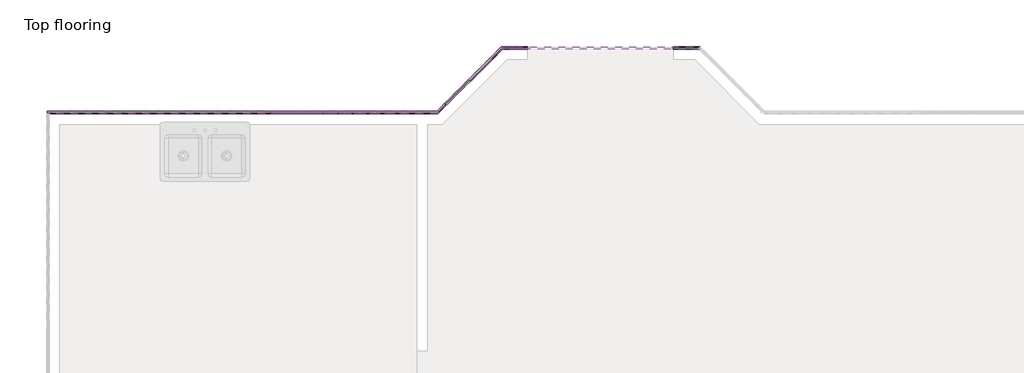
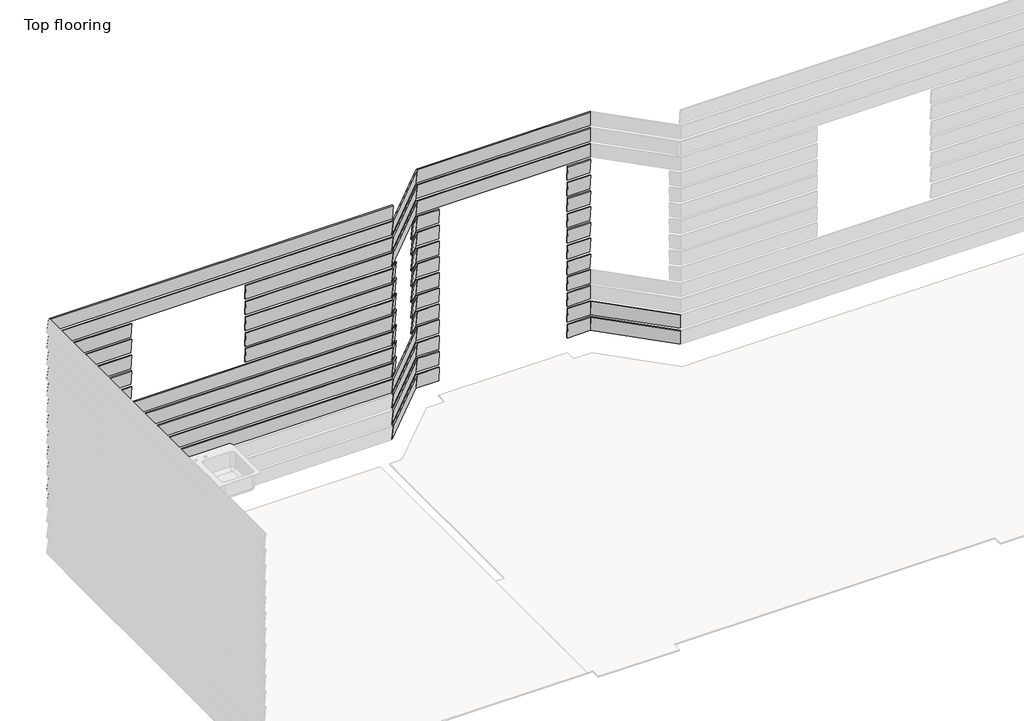
# One storey, part 4 of 5: 42 proxies.
"""IFC4 building model written with IfcOpenShell, lengths in millimetres."""

from ifc_helpers import new_model, si_unit, origin, place, context, project, spatial, faceted_brep, element, save

model = new_model("IFC4")

# Units and contexts
model_context = context("Model", 3, world=origin())
ifc_project = project(units=[si_unit("LENGTHUNIT", "METRE", prefix="MILLI")], contexts=[model_context])

# Site, building, storey
site = spatial("IfcSite", under=ifc_project)
building = spatial("IfcBuilding", under=site)
storey = spatial("IfcBuildingStorey", under=building, Name="Top flooring", Elevation=12.7)

# Proxies
placement = place(None, origin())
element("IfcBuildingElementProxy", 1, Name="Wall Sweeps", at=placement, inside=storey, context=model_context, shape_type="Brep", body=[
    faceted_brep([(-14153.612325, 5231.8645018, 179.3151454), (-14149.4864779, 5221.9038257, 178.429182), (-14143.614829, 5207.7284114, 337.8), (-14147.7406762, 5217.6890875, 338.6859634), (-13544.012325, 5841.4645018, 179.3151454), (-13538.1406762, 5827.2890875, 338.6859634), (-13534.014829, 5817.3284114, 337.8), (-13539.8864779, 5831.5038257, 178.429182)], [[[0, 1, 2, 3]], [[4, 5, 6, 7]], [[1, 0, 4, 7]], [[2, 1, 7, 6]], [[3, 2, 6, 5]], [[0, 3, 5, 4]]]),
])
element("IfcBuildingElementProxy", 2, Name="Wall Sweeps", at=placement, inside=storey, context=model_context, shape_type="Brep", body=[
    faceted_brep([(-14153.612325, 5231.8645018, 357.1151454), (-14149.4864779, 5221.9038257, 356.229182), (-14143.614829, 5207.7284114, 515.6), (-14147.7406762, 5217.6890875, 516.4859634), (-13544.012325, 5841.4645018, 357.1151454), (-13538.1406762, 5827.2890875, 516.4859634), (-13534.014829, 5817.3284114, 515.6), (-13539.8864779, 5831.5038257, 356.229182)], [[[0, 1, 2, 3]], [[4, 5, 6, 7]], [[1, 0, 4, 7]], [[2, 1, 7, 6]], [[3, 2, 6, 5]], [[0, 3, 5, 4]]]),
])
element("IfcBuildingElementProxy", 3, Name="Wall Sweeps", at=placement, inside=storey, context=model_context, shape_type="Brep", body=[
    faceted_brep([(-14153.612325, 5231.8645018, 534.9151454), (-14149.4864779, 5221.9038257, 534.029182), (-14143.614829, 5207.7284114, 693.4), (-14147.7406762, 5217.6890875, 694.2859634), (-13544.012325, 5841.4645018, 534.9151454), (-13538.1406762, 5827.2890875, 694.2859634), (-13534.014829, 5817.3284114, 693.4), (-13539.8864779, 5831.5038257, 534.029182)], [[[0, 1, 2, 3]], [[4, 5, 6, 7]], [[1, 0, 4, 7]], [[2, 1, 7, 6]], [[3, 2, 6, 5]], [[0, 3, 5, 4]]]),
])
element("IfcBuildingElementProxy", 4, Name="Wall Sweeps", at=placement, inside=storey, context=model_context, shape_type="Brep", body=[
    faceted_brep([(-14153.612325, 5231.8645018, 712.7151454), (-14149.4864779, 5221.9038257, 711.829182), (-14143.614829, 5207.7284114, 871.2), (-14147.7406762, 5217.6890875, 872.0859634), (-13544.012325, 5841.4645018, 712.7151454), (-13538.1406762, 5827.2890875, 872.0859634), (-13534.014829, 5817.3284114, 871.2), (-13539.8864779, 5831.5038257, 711.829182)], [[[0, 1, 2, 3]], [[4, 5, 6, 7]], [[1, 0, 4, 7]], [[2, 1, 7, 6]], [[3, 2, 6, 5]], [[0, 3, 5, 4]]]),
])
element("IfcBuildingElementProxy", 5, Name="Wall Sweeps", at=placement, inside=storey, context=model_context, shape_type="Brep", body=[
    faceted_brep([(-13649.8960469, 5735.5807799, 890.5151454), (-13642.8527853, 5728.5375183, 889.629182), (-13632.8292537, 5718.5139867, 1049.0), (-13639.8725153, 5725.5572483, 1049.8859634), (-13544.012325, 5841.4645018, 890.5151454), (-13538.1406762, 5827.2890875, 1049.8859634), (-13534.014829, 5817.3284114, 1049.0), (-13539.8864779, 5831.5038257, 889.629182)], [[[0, 1, 2, 3]], [[4, 5, 6, 7]], [[1, 0, 4, 7]], [[2, 1, 7, 6]], [[3, 2, 6, 5]], [[0, 3, 5, 4]]]),
    faceted_brep([(-14153.612325, 5231.8645018, 890.5151454), (-14149.4864779, 5221.9038257, 889.629182), (-14143.614829, 5207.7284114, 1049.0), (-14147.7406762, 5217.6890875, 1049.8859634), (-14080.9483407, 5304.5284861, 890.5151454), (-14070.9248092, 5294.5049545, 1049.8859634), (-14063.8815475, 5287.4616929, 1049.0), (-14073.9050791, 5297.4852245, 889.629182)], [[[0, 1, 2, 3]], [[4, 5, 6, 7]], [[1, 0, 4, 7]], [[2, 1, 7, 6]], [[3, 2, 6, 5]], [[0, 3, 5, 4]]]),
])
element("IfcBuildingElementProxy", 6, Name="Wall Sweeps", at=placement, inside=storey, context=model_context, shape_type="Brep", body=[
    faceted_brep([(-13649.8960469, 5735.5807799, 1068.3151454), (-13642.8527853, 5728.5375183, 1067.429182), (-13632.8292537, 5718.5139867, 1226.8), (-13639.8725153, 5725.5572483, 1227.6859634), (-13544.012325, 5841.4645018, 1068.3151454), (-13538.1406762, 5827.2890875, 1227.6859634), (-13534.014829, 5817.3284114, 1226.8), (-13539.8864779, 5831.5038257, 1067.429182)], [[[0, 1, 2, 3]], [[4, 5, 6, 7]], [[1, 0, 4, 7]], [[2, 1, 7, 6]], [[3, 2, 6, 5]], [[0, 3, 5, 4]]]),
    faceted_brep([(-14153.612325, 5231.8645018, 1068.3151454), (-14149.4864779, 5221.9038257, 1067.429182), (-14143.614829, 5207.7284114, 1226.8), (-14147.7406762, 5217.6890875, 1227.6859634), (-14080.9483407, 5304.5284861, 1068.3151454), (-14070.9248092, 5294.5049545, 1227.6859634), (-14063.8815475, 5287.4616929, 1226.8), (-14073.9050791, 5297.4852245, 1067.429182)], [[[0, 1, 2, 3]], [[4, 5, 6, 7]], [[1, 0, 4, 7]], [[2, 1, 7, 6]], [[3, 2, 6, 5]], [[0, 3, 5, 4]]]),
])
element("IfcBuildingElementProxy", 7, Name="Wall Sweeps", at=placement, inside=storey, context=model_context, shape_type="Brep", body=[
    faceted_brep([(-13649.8960469, 5735.5807799, 1246.1151454), (-13642.8527853, 5728.5375183, 1245.229182), (-13632.8292537, 5718.5139867, 1404.6), (-13639.8725153, 5725.5572483, 1405.4859634), (-13544.012325, 5841.4645018, 1246.1151454), (-13538.1406762, 5827.2890875, 1405.4859634), (-13534.014829, 5817.3284114, 1404.6), (-13539.8864779, 5831.5038257, 1245.229182)], [[[0, 1, 2, 3]], [[4, 5, 6, 7]], [[1, 0, 4, 7]], [[2, 1, 7, 6]], [[3, 2, 6, 5]], [[0, 3, 5, 4]]]),
    faceted_brep([(-14153.612325, 5231.8645018, 1246.1151454), (-14149.4864779, 5221.9038257, 1245.229182), (-14143.614829, 5207.7284114, 1404.6), (-14147.7406762, 5217.6890875, 1405.4859634), (-14080.9483407, 5304.5284861, 1246.1151454), (-14070.9248092, 5294.5049545, 1405.4859634), (-14063.8815475, 5287.4616929, 1404.6), (-14073.9050791, 5297.4852245, 1245.229182)], [[[0, 1, 2, 3]], [[4, 5, 6, 7]], [[1, 0, 4, 7]], [[2, 1, 7, 6]], [[3, 2, 6, 5]], [[0, 3, 5, 4]]]),
])
element("IfcBuildingElementProxy", 8, Name="Wall Sweeps", at=placement, inside=storey, context=model_context, shape_type="Brep", body=[
    faceted_brep([(-13649.8960469, 5735.5807799, 1423.9151454), (-13642.8527853, 5728.5375183, 1423.029182), (-13632.8292537, 5718.5139867, 1582.4), (-13639.8725153, 5725.5572483, 1583.2859634), (-13544.012325, 5841.4645018, 1423.9151454), (-13538.1406762, 5827.2890875, 1583.2859634), (-13534.014829, 5817.3284114, 1582.4), (-13539.8864779, 5831.5038257, 1423.029182)], [[[0, 1, 2, 3]], [[4, 5, 6, 7]], [[1, 0, 4, 7]], [[2, 1, 7, 6]], [[3, 2, 6, 5]], [[0, 3, 5, 4]]]),
    faceted_brep([(-14153.612325, 5231.8645018, 1423.9151454), (-14149.4864779, 5221.9038257, 1423.029182), (-14143.614829, 5207.7284114, 1582.4), (-14147.7406762, 5217.6890875, 1583.2859634), (-14080.9483407, 5304.5284861, 1423.9151454), (-14070.9248092, 5294.5049545, 1583.2859634), (-14063.8815475, 5287.4616929, 1582.4), (-14073.9050791, 5297.4852245, 1423.029182)], [[[0, 1, 2, 3]], [[4, 5, 6, 7]], [[1, 0, 4, 7]], [[2, 1, 7, 6]], [[3, 2, 6, 5]], [[0, 3, 5, 4]]]),
])
element("IfcBuildingElementProxy", 9, Name="Wall Sweeps", at=placement, inside=storey, context=model_context, shape_type="Brep", body=[
    faceted_brep([(-13649.8960469, 5735.5807799, 1601.7151454), (-13642.8527853, 5728.5375183, 1600.829182), (-13632.8292537, 5718.5139867, 1760.2), (-13639.8725153, 5725.5572483, 1761.0859634), (-13544.012325, 5841.4645018, 1601.7151454), (-13538.1406762, 5827.2890875, 1761.0859634), (-13534.014829, 5817.3284114, 1760.2), (-13539.8864779, 5831.5038257, 1600.829182)], [[[0, 1, 2, 3]], [[4, 5, 6, 7]], [[1, 0, 4, 7]], [[2, 1, 7, 6]], [[3, 2, 6, 5]], [[0, 3, 5, 4]]]),
    faceted_brep([(-14153.612325, 5231.8645018, 1601.7151454), (-14149.4864779, 5221.9038257, 1600.829182), (-14143.614829, 5207.7284114, 1760.2), (-14147.7406762, 5217.6890875, 1761.0859634), (-14080.9483407, 5304.5284861, 1601.7151454), (-14070.9248092, 5294.5049545, 1761.0859634), (-14063.8815475, 5287.4616929, 1760.2), (-14073.9050791, 5297.4852245, 1600.829182)], [[[0, 1, 2, 3]], [[4, 5, 6, 7]], [[1, 0, 4, 7]], [[2, 1, 7, 6]], [[3, 2, 6, 5]], [[0, 3, 5, 4]]]),
])
element("IfcBuildingElementProxy", 10, Name="Wall Sweeps", at=placement, inside=storey, context=model_context, shape_type="Brep", body=[
    faceted_brep([(-13649.8960469, 5735.5807799, 1779.5151454), (-13642.8527853, 5728.5375183, 1778.629182), (-13632.8292537, 5718.5139867, 1938.0), (-13639.8725153, 5725.5572483, 1938.8859634), (-13544.012325, 5841.4645018, 1779.5151454), (-13538.1406762, 5827.2890875, 1938.8859634), (-13534.014829, 5817.3284114, 1938.0), (-13539.8864779, 5831.5038257, 1778.629182)], [[[0, 1, 2, 3]], [[4, 5, 6, 7]], [[1, 0, 4, 7]], [[2, 1, 7, 6]], [[3, 2, 6, 5]], [[0, 3, 5, 4]]]),
    faceted_brep([(-14153.612325, 5231.8645018, 1779.5151454), (-14149.4864779, 5221.9038257, 1778.629182), (-14143.614829, 5207.7284114, 1938.0), (-14147.7406762, 5217.6890875, 1938.8859634), (-14080.9483407, 5304.5284861, 1779.5151454), (-14070.9248092, 5294.5049545, 1938.8859634), (-14063.8815475, 5287.4616929, 1938.0), (-14073.9050791, 5297.4852245, 1778.629182)], [[[0, 1, 2, 3]], [[4, 5, 6, 7]], [[1, 0, 4, 7]], [[2, 1, 7, 6]], [[3, 2, 6, 5]], [[0, 3, 5, 4]]]),
])
element("IfcBuildingElementProxy", 11, Name="Wall Sweeps", at=placement, inside=storey, context=model_context, shape_type="Brep", body=[
    faceted_brep([(-13649.8960469, 5735.5807799, 1957.3151454), (-13642.8527853, 5728.5375183, 1956.429182), (-13632.8292537, 5718.5139867, 2115.8), (-13639.8725153, 5725.5572483, 2116.6859634), (-13544.012325, 5841.4645018, 1957.3151454), (-13538.1406762, 5827.2890875, 2116.6859634), (-13534.014829, 5817.3284114, 2115.8), (-13539.8864779, 5831.5038257, 1956.429182)], [[[0, 1, 2, 3]], [[4, 5, 6, 7]], [[1, 0, 4, 7]], [[2, 1, 7, 6]], [[3, 2, 6, 5]], [[0, 3, 5, 4]]]),
    faceted_brep([(-14153.612325, 5231.8645018, 1957.3151454), (-14149.4864779, 5221.9038257, 1956.429182), (-14143.614829, 5207.7284114, 2115.8), (-14147.7406762, 5217.6890875, 2116.6859634), (-14080.9483407, 5304.5284861, 1957.3151454), (-14070.9248092, 5294.5049545, 2116.6859634), (-14063.8815475, 5287.4616929, 2115.8), (-14073.9050791, 5297.4852245, 1956.429182)], [[[0, 1, 2, 3]], [[4, 5, 6, 7]], [[1, 0, 4, 7]], [[2, 1, 7, 6]], [[3, 2, 6, 5]], [[0, 3, 5, 4]]]),
])
element("IfcBuildingElementProxy", 12, Name="Wall Sweeps", at=placement, inside=storey, context=model_context, shape_type="Brep", body=[
    faceted_brep([(-14153.612325, 5231.8645018, 2135.1151454), (-14149.4864779, 5221.9038257, 2134.229182), (-14143.614829, 5207.7284114, 2293.6), (-14147.7406762, 5217.6890875, 2294.4859634), (-13544.012325, 5841.4645018, 2135.1151454), (-13538.1406762, 5827.2890875, 2294.4859634), (-13534.014829, 5817.3284114, 2293.6), (-13539.8864779, 5831.5038257, 2134.229182)], [[[0, 1, 2, 3]], [[4, 5, 6, 7]], [[1, 0, 4, 7]], [[2, 1, 7, 6]], [[3, 2, 6, 5]], [[0, 3, 5, 4]]]),
])
element("IfcBuildingElementProxy", 13, Name="Wall Sweeps", at=placement, inside=storey, context=model_context, shape_type="Brep", body=[
    faceted_brep([(-13544.012325, 5841.4645018, 179.3151454), (-13539.8864779, 5831.5038257, 178.429182), (-13534.014829, 5817.3284114, 337.8), (-13538.1406762, 5827.2890875, 338.6859634), (-13297.0301791, 5841.4645018, 179.3151454), (-13297.0301791, 5827.2890875, 338.6859634), (-13297.0301791, 5817.3284114, 337.8), (-13297.0301791, 5831.5038257, 178.429182)], [[[0, 1, 2, 3]], [[4, 5, 6, 7]], [[1, 0, 4, 7]], [[2, 1, 7, 6]], [[3, 2, 6, 5]], [[0, 3, 5, 4]]]),
    faceted_brep([(-11925.4301791, 5841.4645018, 179.3151454), (-11925.4301791, 5831.5038257, 178.429182), (-11925.4301791, 5817.3284114, 337.8), (-11925.4301791, 5827.2890875, 338.6859634), (-11674.1752841, 5841.4645018, 179.3151454), (-11680.0469329, 5827.2890875, 338.6859634), (-11684.1727801, 5817.3284114, 337.8), (-11678.3011312, 5831.5038257, 178.429182)], [[[0, 1, 2, 3]], [[4, 5, 6, 7]], [[1, 0, 4, 7]], [[2, 1, 7, 6]], [[3, 2, 6, 5]], [[0, 3, 5, 4]]]),
])
element("IfcBuildingElementProxy", 14, Name="Wall Sweeps", at=placement, inside=storey, context=model_context, shape_type="Brep", body=[
    faceted_brep([(-13544.012325, 5841.4645018, 357.1151454), (-13539.8864779, 5831.5038257, 356.229182), (-13534.014829, 5817.3284114, 515.6), (-13538.1406762, 5827.2890875, 516.4859634), (-13297.0301791, 5841.4645018, 357.1151454), (-13297.0301791, 5827.2890875, 516.4859634), (-13297.0301791, 5817.3284114, 515.6), (-13297.0301791, 5831.5038257, 356.229182)], [[[0, 1, 2, 3]], [[4, 5, 6, 7]], [[1, 0, 4, 7]], [[2, 1, 7, 6]], [[3, 2, 6, 5]], [[0, 3, 5, 4]]]),
    faceted_brep([(-11925.4301791, 5841.4645018, 357.1151454), (-11925.4301791, 5831.5038257, 356.229182), (-11925.4301791, 5817.3284114, 515.6), (-11925.4301791, 5827.2890875, 516.4859634), (-11674.1752841, 5841.4645018, 357.1151454), (-11680.0469329, 5827.2890875, 516.4859634), (-11684.1727801, 5817.3284114, 515.6), (-11678.3011312, 5831.5038257, 356.229182)], [[[0, 1, 2, 3]], [[4, 5, 6, 7]], [[1, 0, 4, 7]], [[2, 1, 7, 6]], [[3, 2, 6, 5]], [[0, 3, 5, 4]]]),
])
element("IfcBuildingElementProxy", 15, Name="Wall Sweeps", at=placement, inside=storey, context=model_context, shape_type="Brep", body=[
    faceted_brep([(-13544.012325, 5841.4645018, 534.9151454), (-13539.8864779, 5831.5038257, 534.029182), (-13534.014829, 5817.3284114, 693.4), (-13538.1406762, 5827.2890875, 694.2859634), (-13297.0301791, 5841.4645018, 534.9151454), (-13297.0301791, 5827.2890875, 694.2859634), (-13297.0301791, 5817.3284114, 693.4), (-13297.0301791, 5831.5038257, 534.029182)], [[[0, 1, 2, 3]], [[4, 5, 6, 7]], [[1, 0, 4, 7]], [[2, 1, 7, 6]], [[3, 2, 6, 5]], [[0, 3, 5, 4]]]),
    faceted_brep([(-11925.4301791, 5841.4645018, 534.9151454), (-11925.4301791, 5831.5038257, 534.029182), (-11925.4301791, 5817.3284114, 693.4), (-11925.4301791, 5827.2890875, 694.2859634), (-11674.1752841, 5841.4645018, 534.9151454), (-11680.0469329, 5827.2890875, 694.2859634), (-11684.1727801, 5817.3284114, 693.4), (-11678.3011312, 5831.5038257, 534.029182)], [[[0, 1, 2, 3]], [[4, 5, 6, 7]], [[1, 0, 4, 7]], [[2, 1, 7, 6]], [[3, 2, 6, 5]], [[0, 3, 5, 4]]]),
])
element("IfcBuildingElementProxy", 16, Name="Wall Sweeps", at=placement, inside=storey, context=model_context, shape_type="Brep", body=[
    faceted_brep([(-13544.012325, 5841.4645018, 712.7151454), (-13539.8864779, 5831.5038257, 711.829182), (-13534.014829, 5817.3284114, 871.2), (-13538.1406762, 5827.2890875, 872.0859634), (-13297.0301791, 5841.4645018, 712.7151454), (-13297.0301791, 5827.2890875, 872.0859634), (-13297.0301791, 5817.3284114, 871.2), (-13297.0301791, 5831.5038257, 711.829182)], [[[0, 1, 2, 3]], [[4, 5, 6, 7]], [[1, 0, 4, 7]], [[2, 1, 7, 6]], [[3, 2, 6, 5]], [[0, 3, 5, 4]]]),
    faceted_brep([(-11925.4301791, 5841.4645018, 712.7151454), (-11925.4301791, 5831.5038257, 711.829182), (-11925.4301791, 5817.3284114, 871.2), (-11925.4301791, 5827.2890875, 872.0859634), (-11674.1752841, 5841.4645018, 712.7151454), (-11680.0469329, 5827.2890875, 872.0859634), (-11684.1727801, 5817.3284114, 871.2), (-11678.3011312, 5831.5038257, 711.829182)], [[[0, 1, 2, 3]], [[4, 5, 6, 7]], [[1, 0, 4, 7]], [[2, 1, 7, 6]], [[3, 2, 6, 5]], [[0, 3, 5, 4]]]),
])
element("IfcBuildingElementProxy", 17, Name="Wall Sweeps", at=placement, inside=storey, context=model_context, shape_type="Brep", body=[
    faceted_brep([(-13544.012325, 5841.4645018, 890.5151454), (-13539.8864779, 5831.5038257, 889.629182), (-13534.014829, 5817.3284114, 1049.0), (-13538.1406762, 5827.2890875, 1049.8859634), (-13297.0301791, 5841.4645018, 890.5151454), (-13297.0301791, 5827.2890875, 1049.8859634), (-13297.0301791, 5817.3284114, 1049.0), (-13297.0301791, 5831.5038257, 889.629182)], [[[0, 1, 2, 3]], [[4, 5, 6, 7]], [[1, 0, 4, 7]], [[2, 1, 7, 6]], [[3, 2, 6, 5]], [[0, 3, 5, 4]]]),
    faceted_brep([(-11925.4301791, 5841.4645018, 890.5151454), (-11925.4301791, 5831.5038257, 889.629182), (-11925.4301791, 5817.3284114, 1049.0), (-11925.4301791, 5827.2890875, 1049.8859634), (-11684.1727801, 5841.4645018, 890.5151454), (-11684.1727801, 5827.2890875, 1049.8859634), (-11684.1727801, 5817.3284114, 1049.0), (-11684.1727801, 5831.5038257, 889.629182)], [[[0, 1, 2, 3]], [[4, 5, 6, 7]], [[1, 0, 4, 7]], [[2, 1, 7, 6]], [[3, 2, 6, 5]], [[0, 3, 5, 4]]]),
])
element("IfcBuildingElementProxy", 18, Name="Wall Sweeps", at=placement, inside=storey, context=model_context, shape_type="Brep", body=[
    faceted_brep([(-13544.012325, 5841.4645018, 1068.3151454), (-13539.8864779, 5831.5038257, 1067.429182), (-13534.014829, 5817.3284114, 1226.8), (-13538.1406762, 5827.2890875, 1227.6859634), (-13297.0301791, 5841.4645018, 1068.3151454), (-13297.0301791, 5827.2890875, 1227.6859634), (-13297.0301791, 5817.3284114, 1226.8), (-13297.0301791, 5831.5038257, 1067.429182)], [[[0, 1, 2, 3]], [[4, 5, 6, 7]], [[1, 0, 4, 7]], [[2, 1, 7, 6]], [[3, 2, 6, 5]], [[0, 3, 5, 4]]]),
    faceted_brep([(-11925.4301791, 5841.4645018, 1068.3151454), (-11925.4301791, 5831.5038257, 1067.429182), (-11925.4301791, 5817.3284114, 1226.8), (-11925.4301791, 5827.2890875, 1227.6859634), (-11684.1727801, 5841.4645018, 1068.3151454), (-11684.1727801, 5827.2890875, 1227.6859634), (-11684.1727801, 5817.3284114, 1226.8), (-11684.1727801, 5831.5038257, 1067.429182)], [[[0, 1, 2, 3]], [[4, 5, 6, 7]], [[1, 0, 4, 7]], [[2, 1, 7, 6]], [[3, 2, 6, 5]], [[0, 3, 5, 4]]]),
])
element("IfcBuildingElementProxy", 19, Name="Wall Sweeps", at=placement, inside=storey, context=model_context, shape_type="Brep", body=[
    faceted_brep([(-13544.012325, 5841.4645018, 1246.1151454), (-13539.8864779, 5831.5038257, 1245.229182), (-13534.014829, 5817.3284114, 1404.6), (-13538.1406762, 5827.2890875, 1405.4859634), (-13297.0301791, 5841.4645018, 1246.1151454), (-13297.0301791, 5827.2890875, 1405.4859634), (-13297.0301791, 5817.3284114, 1404.6), (-13297.0301791, 5831.5038257, 1245.229182)], [[[0, 1, 2, 3]], [[4, 5, 6, 7]], [[1, 0, 4, 7]], [[2, 1, 7, 6]], [[3, 2, 6, 5]], [[0, 3, 5, 4]]]),
    faceted_brep([(-11925.4301791, 5841.4645018, 1246.1151454), (-11925.4301791, 5831.5038257, 1245.229182), (-11925.4301791, 5817.3284114, 1404.6), (-11925.4301791, 5827.2890875, 1405.4859634), (-11684.1727801, 5841.4645018, 1246.1151454), (-11684.1727801, 5827.2890875, 1405.4859634), (-11684.1727801, 5817.3284114, 1404.6), (-11684.1727801, 5831.5038257, 1245.229182)], [[[0, 1, 2, 3]], [[4, 5, 6, 7]], [[1, 0, 4, 7]], [[2, 1, 7, 6]], [[3, 2, 6, 5]], [[0, 3, 5, 4]]]),
])
element("IfcBuildingElementProxy", 20, Name="Wall Sweeps", at=placement, inside=storey, context=model_context, shape_type="Brep", body=[
    faceted_brep([(-13544.012325, 5841.4645018, 1423.9151454), (-13539.8864779, 5831.5038257, 1423.029182), (-13534.014829, 5817.3284114, 1582.4), (-13538.1406762, 5827.2890875, 1583.2859634), (-13297.0301791, 5841.4645018, 1423.9151454), (-13297.0301791, 5827.2890875, 1583.2859634), (-13297.0301791, 5817.3284114, 1582.4), (-13297.0301791, 5831.5038257, 1423.029182)], [[[0, 1, 2, 3]], [[4, 5, 6, 7]], [[1, 0, 4, 7]], [[2, 1, 7, 6]], [[3, 2, 6, 5]], [[0, 3, 5, 4]]]),
    faceted_brep([(-11925.4301791, 5841.4645018, 1423.9151454), (-11925.4301791, 5831.5038257, 1423.029182), (-11925.4301791, 5817.3284114, 1582.4), (-11925.4301791, 5827.2890875, 1583.2859634), (-11684.1727801, 5841.4645018, 1423.9151454), (-11684.1727801, 5827.2890875, 1583.2859634), (-11684.1727801, 5817.3284114, 1582.4), (-11684.1727801, 5831.5038257, 1423.029182)], [[[0, 1, 2, 3]], [[4, 5, 6, 7]], [[1, 0, 4, 7]], [[2, 1, 7, 6]], [[3, 2, 6, 5]], [[0, 3, 5, 4]]]),
])
element("IfcBuildingElementProxy", 21, Name="Wall Sweeps", at=placement, inside=storey, context=model_context, shape_type="Brep", body=[
    faceted_brep([(-13544.012325, 5841.4645018, 1601.7151454), (-13539.8864779, 5831.5038257, 1600.829182), (-13534.014829, 5817.3284114, 1760.2), (-13538.1406762, 5827.2890875, 1761.0859634), (-13297.0301791, 5841.4645018, 1601.7151454), (-13297.0301791, 5827.2890875, 1761.0859634), (-13297.0301791, 5817.3284114, 1760.2), (-13297.0301791, 5831.5038257, 1600.829182)], [[[0, 1, 2, 3]], [[4, 5, 6, 7]], [[1, 0, 4, 7]], [[2, 1, 7, 6]], [[3, 2, 6, 5]], [[0, 3, 5, 4]]]),
    faceted_brep([(-11925.4301791, 5841.4645018, 1601.7151454), (-11925.4301791, 5831.5038257, 1600.829182), (-11925.4301791, 5817.3284114, 1760.2), (-11925.4301791, 5827.2890875, 1761.0859634), (-11684.1727801, 5841.4645018, 1601.7151454), (-11684.1727801, 5827.2890875, 1761.0859634), (-11684.1727801, 5817.3284114, 1760.2), (-11684.1727801, 5831.5038257, 1600.829182)], [[[0, 1, 2, 3]], [[4, 5, 6, 7]], [[1, 0, 4, 7]], [[2, 1, 7, 6]], [[3, 2, 6, 5]], [[0, 3, 5, 4]]]),
])
element("IfcBuildingElementProxy", 22, Name="Wall Sweeps", at=placement, inside=storey, context=model_context, shape_type="Brep", body=[
    faceted_brep([(-13544.012325, 5841.4645018, 1779.5151454), (-13539.8864779, 5831.5038257, 1778.629182), (-13534.014829, 5817.3284114, 1938.0), (-13538.1406762, 5827.2890875, 1938.8859634), (-13297.0301791, 5841.4645018, 1779.5151454), (-13297.0301791, 5827.2890875, 1938.8859634), (-13297.0301791, 5817.3284114, 1938.0), (-13297.0301791, 5831.5038257, 1778.629182)], [[[0, 1, 2, 3]], [[4, 5, 6, 7]], [[1, 0, 4, 7]], [[2, 1, 7, 6]], [[3, 2, 6, 5]], [[0, 3, 5, 4]]]),
    faceted_brep([(-11925.4301791, 5841.4645018, 1779.5151454), (-11925.4301791, 5831.5038257, 1778.629182), (-11925.4301791, 5817.3284114, 1938.0), (-11925.4301791, 5827.2890875, 1938.8859634), (-11684.1727801, 5841.4645018, 1779.5151454), (-11684.1727801, 5827.2890875, 1938.8859634), (-11684.1727801, 5817.3284114, 1938.0), (-11684.1727801, 5831.5038257, 1778.629182)], [[[0, 1, 2, 3]], [[4, 5, 6, 7]], [[1, 0, 4, 7]], [[2, 1, 7, 6]], [[3, 2, 6, 5]], [[0, 3, 5, 4]]]),
])
element("IfcBuildingElementProxy", 23, Name="Wall Sweeps", at=placement, inside=storey, context=model_context, shape_type="Brep", body=[
    faceted_brep([(-13544.012325, 5841.4645018, 1957.3151454), (-13539.8864779, 5831.5038257, 1956.429182), (-13534.014829, 5817.3284114, 2115.8), (-13538.1406762, 5827.2890875, 2116.6859634), (-13297.0301791, 5841.4645018, 1957.3151454), (-13297.0301791, 5827.2890875, 2116.6859634), (-13297.0301791, 5817.3284114, 2115.8), (-13297.0301791, 5831.5038257, 1956.429182)], [[[0, 1, 2, 3]], [[4, 5, 6, 7]], [[1, 0, 4, 7]], [[2, 1, 7, 6]], [[3, 2, 6, 5]], [[0, 3, 5, 4]]]),
    faceted_brep([(-11925.4301791, 5841.4645018, 1957.3151454), (-11925.4301791, 5831.5038257, 1956.429182), (-11925.4301791, 5817.3284114, 2115.8), (-11925.4301791, 5827.2890875, 2116.6859634), (-11684.1727801, 5841.4645018, 1957.3151454), (-11684.1727801, 5827.2890875, 2116.6859634), (-11684.1727801, 5817.3284114, 2115.8), (-11684.1727801, 5831.5038257, 1956.429182)], [[[0, 1, 2, 3]], [[4, 5, 6, 7]], [[1, 0, 4, 7]], [[2, 1, 7, 6]], [[3, 2, 6, 5]], [[0, 3, 5, 4]]]),
])
element("IfcBuildingElementProxy", 24, Name="Wall Sweeps", at=placement, inside=storey, context=model_context, shape_type="Brep", body=[
    faceted_brep([(-13544.012325, 5841.4645018, 2135.1151454), (-13539.8864779, 5831.5038257, 2134.229182), (-13534.014829, 5817.3284114, 2293.6), (-13538.1406762, 5827.2890875, 2294.4859634), (-11674.1752841, 5841.4645018, 2135.1151454), (-11680.0469329, 5827.2890875, 2294.4859634), (-11684.1727801, 5817.3284114, 2293.6), (-11678.3011312, 5831.5038257, 2134.229182)], [[[0, 1, 2, 3]], [[4, 5, 6, 7]], [[1, 0, 4, 7]], [[2, 1, 7, 6]], [[3, 2, 6, 5]], [[0, 3, 5, 4]]]),
])
element("IfcBuildingElementProxy", 25, Name="Wall Sweeps", at=placement, inside=storey, context=model_context, shape_type="Brep", body=[
    faceted_brep([(-11064.5752841, 5231.8645018, 179.3151454), (-11070.4469329, 5217.6890875, 338.6859634), (-11074.5727801, 5207.7284114, 337.8), (-11068.7011312, 5221.9038257, 178.429182), (-11674.1752841, 5841.4645018, 179.3151454), (-11678.3011312, 5831.5038257, 178.429182), (-11684.1727801, 5817.3284114, 337.8), (-11680.0469329, 5827.2890875, 338.6859634)], [[[0, 1, 2, 3]], [[4, 5, 6, 7]], [[1, 0, 4, 7]], [[2, 1, 7, 6]], [[3, 2, 6, 5]], [[0, 3, 5, 4]]]),
])
element("IfcBuildingElementProxy", 26, Name="Wall Sweeps", at=placement, inside=storey, context=model_context, shape_type="Brep", body=[
    faceted_brep([(-11064.5752841, 5231.8645018, 357.1151454), (-11070.4469329, 5217.6890875, 516.4859634), (-11074.5727801, 5207.7284114, 515.6), (-11068.7011312, 5221.9038257, 356.229182), (-11674.1752841, 5841.4645018, 357.1151454), (-11678.3011312, 5831.5038257, 356.229182), (-11684.1727801, 5817.3284114, 515.6), (-11680.0469329, 5827.2890875, 516.4859634)], [[[0, 1, 2, 3]], [[4, 5, 6, 7]], [[1, 0, 4, 7]], [[2, 1, 7, 6]], [[3, 2, 6, 5]], [[0, 3, 5, 4]]]),
])
element("IfcBuildingElementProxy", 27, Name="Wall Sweeps", at=placement, inside=storey, context=model_context, shape_type="Brep", body=[
    faceted_brep([(-17825.3509195, 5231.8645018, 712.7151454), (-17815.3902433, 5221.9038257, 711.829182), (-17801.214829, 5207.7284114, 871.2), (-17811.1755052, 5217.6890875, 872.0859634), (-14153.612325, 5231.8645018, 712.7151454), (-14147.7406762, 5217.6890875, 872.0859634), (-14143.614829, 5207.7284114, 871.2), (-14149.4864779, 5221.9038257, 711.829182)], [[[0, 1, 2, 3]], [[4, 5, 6, 7]], [[1, 0, 4, 7]], [[2, 1, 7, 6]], [[3, 2, 6, 5]], [[0, 3, 5, 4]]]),
])
element("IfcBuildingElementProxy", 28, Name="Wall Sweeps", at=placement, inside=storey, context=model_context, shape_type="Brep", body=[
    faceted_brep([(-17825.3509195, 5231.8645018, 890.5151454), (-17815.3902433, 5221.9038257, 889.629182), (-17801.214829, 5207.7284114, 1049.0), (-17811.1755052, 5217.6890875, 1049.8859634), (-14153.612325, 5231.8645018, 890.5151454), (-14147.7406762, 5217.6890875, 1049.8859634), (-14143.614829, 5207.7284114, 1049.0), (-14149.4864779, 5221.9038257, 889.629182)], [[[0, 1, 2, 3]], [[4, 5, 6, 7]], [[1, 0, 4, 7]], [[2, 1, 7, 6]], [[3, 2, 6, 5]], [[0, 3, 5, 4]]]),
])
element("IfcBuildingElementProxy", 29, Name="Wall Sweeps", at=placement, inside=storey, context=model_context, shape_type="Brep", body=[
    faceted_brep([(-17825.3509195, 5231.8645018, 1068.3151454), (-17815.3902433, 5221.9038257, 1067.429182), (-17801.214829, 5207.7284114, 1226.8), (-17811.1755052, 5217.6890875, 1227.6859634), (-14153.612325, 5231.8645018, 1068.3151454), (-14147.7406762, 5217.6890875, 1227.6859634), (-14143.614829, 5207.7284114, 1226.8), (-14149.4864779, 5221.9038257, 1067.429182)], [[[0, 1, 2, 3]], [[4, 5, 6, 7]], [[1, 0, 4, 7]], [[2, 1, 7, 6]], [[3, 2, 6, 5]], [[0, 3, 5, 4]]]),
])
element("IfcBuildingElementProxy", 30, Name="Wall Sweeps", at=placement, inside=storey, context=model_context, shape_type="Brep", body=[
    faceted_brep([(-17825.3509195, 5231.8645018, 1246.1151454), (-17815.3902433, 5221.9038257, 1245.229182), (-17801.214829, 5207.7284114, 1404.6), (-17811.1755052, 5217.6890875, 1405.4859634), (-14153.612325, 5231.8645018, 1246.1151454), (-14147.7406762, 5217.6890875, 1405.4859634), (-14143.614829, 5207.7284114, 1404.6), (-14149.4864779, 5221.9038257, 1245.229182)], [[[0, 1, 2, 3]], [[4, 5, 6, 7]], [[1, 0, 4, 7]], [[2, 1, 7, 6]], [[3, 2, 6, 5]], [[0, 3, 5, 4]]]),
])
element("IfcBuildingElementProxy", 31, Name="Wall Sweeps", at=placement, inside=storey, context=model_context, shape_type="Brep", body=[
    faceted_brep([(-17825.3509195, 5231.8645018, 1423.9151454), (-17815.3902433, 5221.9038257, 1423.029182), (-17801.214829, 5207.7284114, 1582.4), (-17811.1755052, 5217.6890875, 1583.2859634), (-14153.612325, 5231.8645018, 1423.9151454), (-14147.7406762, 5217.6890875, 1583.2859634), (-14143.614829, 5207.7284114, 1582.4), (-14149.4864779, 5221.9038257, 1423.029182)], [[[0, 1, 2, 3]], [[4, 5, 6, 7]], [[1, 0, 4, 7]], [[2, 1, 7, 6]], [[3, 2, 6, 5]], [[0, 3, 5, 4]]]),
])
element("IfcBuildingElementProxy", 32, Name="Wall Sweeps", at=placement, inside=storey, context=model_context, shape_type="Brep", body=[
    faceted_brep([(-17825.3509195, 5231.8645018, 1601.7151454), (-17815.3902433, 5221.9038257, 1600.829182), (-17801.214829, 5207.7284114, 1760.2), (-17811.1755052, 5217.6890875, 1761.0859634), (-16931.7167223, 5231.8645018, 1601.7151454), (-16931.7167223, 5217.6890875, 1761.0859634), (-16931.7167223, 5207.7284114, 1760.2), (-16931.7167223, 5221.9038257, 1600.829182)], [[[0, 1, 2, 3]], [[4, 5, 6, 7]], [[1, 0, 4, 7]], [[2, 1, 7, 6]], [[3, 2, 6, 5]], [[0, 3, 5, 4]]]),
    faceted_brep([(-15712.5167223, 5231.8645018, 1601.7151454), (-15712.5167223, 5221.9038257, 1600.829182), (-15712.5167223, 5207.7284114, 1760.2), (-15712.5167223, 5217.6890875, 1761.0859634), (-14153.612325, 5231.8645018, 1601.7151454), (-14147.7406762, 5217.6890875, 1761.0859634), (-14143.614829, 5207.7284114, 1760.2), (-14149.4864779, 5221.9038257, 1600.829182)], [[[0, 1, 2, 3]], [[4, 5, 6, 7]], [[1, 0, 4, 7]], [[2, 1, 7, 6]], [[3, 2, 6, 5]], [[0, 3, 5, 4]]]),
])
element("IfcBuildingElementProxy", 33, Name="Wall Sweeps", at=placement, inside=storey, context=model_context, shape_type="Brep", body=[
    faceted_brep([(-17825.3509195, 5231.8645018, 1779.5151454), (-17815.3902433, 5221.9038257, 1778.629182), (-17801.214829, 5207.7284114, 1938.0), (-17811.1755052, 5217.6890875, 1938.8859634), (-16931.7167223, 5231.8645018, 1779.5151454), (-16931.7167223, 5217.6890875, 1938.8859634), (-16931.7167223, 5207.7284114, 1938.0), (-16931.7167223, 5221.9038257, 1778.629182)], [[[0, 1, 2, 3]], [[4, 5, 6, 7]], [[1, 0, 4, 7]], [[2, 1, 7, 6]], [[3, 2, 6, 5]], [[0, 3, 5, 4]]]),
    faceted_brep([(-15712.5167223, 5231.8645018, 1779.5151454), (-15712.5167223, 5221.9038257, 1778.629182), (-15712.5167223, 5207.7284114, 1938.0), (-15712.5167223, 5217.6890875, 1938.8859634), (-14153.612325, 5231.8645018, 1779.5151454), (-14147.7406762, 5217.6890875, 1938.8859634), (-14143.614829, 5207.7284114, 1938.0), (-14149.4864779, 5221.9038257, 1778.629182)], [[[0, 1, 2, 3]], [[4, 5, 6, 7]], [[1, 0, 4, 7]], [[2, 1, 7, 6]], [[3, 2, 6, 5]], [[0, 3, 5, 4]]]),
])
element("IfcBuildingElementProxy", 34, Name="Wall Sweeps", at=placement, inside=storey, context=model_context, shape_type="Brep", body=[
    faceted_brep([(-15712.5167223, 5231.8645018, 1957.3151454), (-15712.5167223, 5221.9038257, 1956.429182), (-15712.5167223, 5207.7284114, 2115.8), (-15712.5167223, 5217.6890875, 2116.6859634), (-14153.612325, 5231.8645018, 1957.3151454), (-14147.7406762, 5217.6890875, 2116.6859634), (-14143.614829, 5207.7284114, 2115.8), (-14149.4864779, 5221.9038257, 1956.429182)], [[[0, 1, 2, 3]], [[4, 5, 6, 7]], [[1, 0, 4, 7]], [[2, 1, 7, 6]], [[3, 2, 6, 5]], [[0, 3, 5, 4]]]),
    faceted_brep([(-17825.3509195, 5231.8645018, 1957.3151454), (-17815.3902433, 5221.9038257, 1956.429182), (-17801.214829, 5207.7284114, 2115.8), (-17811.1755052, 5217.6890875, 2116.6859634), (-16931.7167223, 5231.8645018, 1957.3151454), (-16931.7167223, 5217.6890875, 2116.6859634), (-16931.7167223, 5207.7284114, 2115.8), (-16931.7167223, 5221.9038257, 1956.429182)], [[[0, 1, 2, 3]], [[4, 5, 6, 7]], [[1, 0, 4, 7]], [[2, 1, 7, 6]], [[3, 2, 6, 5]], [[0, 3, 5, 4]]]),
])
element("IfcBuildingElementProxy", 35, Name="Wall Sweeps", at=placement, inside=storey, context=model_context, shape_type="Brep", body=[
    faceted_brep([(-15712.5167223, 5231.8645018, 2135.1151454), (-15712.5167223, 5221.9038257, 2134.229182), (-15712.5167223, 5207.7284114, 2293.6), (-15712.5167223, 5217.6890875, 2294.4859634), (-14153.612325, 5231.8645018, 2135.1151454), (-14147.7406762, 5217.6890875, 2294.4859634), (-14143.614829, 5207.7284114, 2293.6), (-14149.4864779, 5221.9038257, 2134.229182)], [[[0, 1, 2, 3]], [[4, 5, 6, 7]], [[1, 0, 4, 7]], [[2, 1, 7, 6]], [[3, 2, 6, 5]], [[0, 3, 5, 4]]]),
    faceted_brep([(-17825.3509195, 5231.8645018, 2135.1151454), (-17815.3902433, 5221.9038257, 2134.229182), (-17801.214829, 5207.7284114, 2293.6), (-17811.1755052, 5217.6890875, 2294.4859634), (-16931.7167223, 5231.8645018, 2135.1151454), (-16931.7167223, 5217.6890875, 2294.4859634), (-16931.7167223, 5207.7284114, 2293.6), (-16931.7167223, 5221.9038257, 2134.229182)], [[[0, 1, 2, 3]], [[4, 5, 6, 7]], [[1, 0, 4, 7]], [[2, 1, 7, 6]], [[3, 2, 6, 5]], [[0, 3, 5, 4]]]),
])
element("IfcBuildingElementProxy", 36, Name="Wall Sweeps", at=placement, inside=storey, context=model_context, shape_type="Brep", body=[
    faceted_brep([(-15712.5167223, 5231.8645018, 2312.9151454), (-15712.5167223, 5221.9038257, 2312.029182), (-15712.5167223, 5207.7284114, 2471.4), (-15712.5167223, 5217.6890875, 2472.2859634), (-14153.612325, 5231.8645018, 2312.9151454), (-14147.7406762, 5217.6890875, 2472.2859634), (-14143.614829, 5207.7284114, 2471.4), (-14149.4864779, 5221.9038257, 2312.029182)], [[[0, 1, 2, 3]], [[4, 5, 6, 7]], [[1, 0, 4, 7]], [[2, 1, 7, 6]], [[3, 2, 6, 5]], [[0, 3, 5, 4]]]),
    faceted_brep([(-17825.3509195, 5231.8645018, 2312.9151454), (-17815.3902433, 5221.9038257, 2312.029182), (-17801.214829, 5207.7284114, 2471.4), (-17811.1755052, 5217.6890875, 2472.2859634), (-16931.7167223, 5231.8645018, 2312.9151454), (-16931.7167223, 5217.6890875, 2472.2859634), (-16931.7167223, 5207.7284114, 2471.4), (-16931.7167223, 5221.9038257, 2312.029182)], [[[0, 1, 2, 3]], [[4, 5, 6, 7]], [[1, 0, 4, 7]], [[2, 1, 7, 6]], [[3, 2, 6, 5]], [[0, 3, 5, 4]]]),
])
element("IfcBuildingElementProxy", 37, Name="Wall Sweeps", at=placement, inside=storey, context=model_context, shape_type="Brep", body=[
    faceted_brep([(-17825.3509195, 5231.8645018, 2490.7151454), (-17815.3902433, 5221.9038257, 2489.829182), (-17801.214829, 5207.7284114, 2649.2), (-17811.1755052, 5217.6890875, 2650.0859634), (-14153.612325, 5231.8645018, 2490.7151454), (-14147.7406762, 5217.6890875, 2650.0859634), (-14143.614829, 5207.7284114, 2649.2), (-14149.4864779, 5221.9038257, 2489.829182)], [[[0, 1, 2, 3]], [[4, 5, 6, 7]], [[1, 0, 4, 7]], [[2, 1, 7, 6]], [[3, 2, 6, 5]], [[0, 3, 5, 4]]]),
])
element("IfcBuildingElementProxy", 38, Name="Wall Sweeps", at=placement, inside=storey, context=model_context, shape_type="Brep", body=[
    faceted_brep([(-17825.3509195, 5231.8645018, 2668.5151454), (-17815.3902433, 5221.9038257, 2667.629182), (-17801.214829, 5207.7284114, 2827.0), (-17811.1755052, 5217.6890875, 2827.8859634), (-14143.614829, 5231.8645018, 2668.5151454), (-14143.614829, 5217.6890875, 2827.8859634), (-14143.614829, 5207.7284114, 2827.0), (-14143.614829, 5221.9038257, 2667.629182)], [[[0, 1, 2, 3]], [[4, 5, 6, 7]], [[1, 0, 4, 7]], [[2, 1, 7, 6]], [[3, 2, 6, 5]], [[0, 3, 5, 4]]]),
])
element("IfcBuildingElementProxy", 39, Name="Wall Sweeps", at=placement, inside=storey, context=model_context, shape_type="Brep", body=[
    faceted_brep([(-14153.612325, 5231.8645018, 2312.9151454), (-14149.4864779, 5221.9038257, 2312.029182), (-14143.614829, 5207.7284114, 2471.4), (-14147.7406762, 5217.6890875, 2472.2859634), (-13544.012325, 5841.4645018, 2312.9151454), (-13538.1406762, 5827.2890875, 2472.2859634), (-13534.014829, 5817.3284114, 2471.4), (-13539.8864779, 5831.5038257, 2312.029182)], [[[0, 1, 2, 3]], [[4, 5, 6, 7]], [[1, 0, 4, 7]], [[2, 1, 7, 6]], [[3, 2, 6, 5]], [[0, 3, 5, 4]]]),
])
element("IfcBuildingElementProxy", 40, Name="Wall Sweeps", at=placement, inside=storey, context=model_context, shape_type="Brep", body=[
    faceted_brep([(-14153.612325, 5231.8645018, 2490.7151454), (-14149.4864779, 5221.9038257, 2489.829182), (-14143.614829, 5207.7284114, 2649.2), (-14147.7406762, 5217.6890875, 2650.0859634), (-13544.012325, 5841.4645018, 2490.7151454), (-13538.1406762, 5827.2890875, 2650.0859634), (-13534.014829, 5817.3284114, 2649.2), (-13539.8864779, 5831.5038257, 2489.829182)], [[[0, 1, 2, 3]], [[4, 5, 6, 7]], [[1, 0, 4, 7]], [[2, 1, 7, 6]], [[3, 2, 6, 5]], [[0, 3, 5, 4]]]),
])
element("IfcBuildingElementProxy", 41, Name="Wall Sweeps", at=placement, inside=storey, context=model_context, shape_type="Brep", body=[
    faceted_brep([(-13544.012325, 5841.4645018, 2312.9151454), (-13539.8864779, 5831.5038257, 2312.029182), (-13534.014829, 5817.3284114, 2471.4), (-13538.1406762, 5827.2890875, 2472.2859634), (-11674.1752841, 5841.4645018, 2312.9151454), (-11680.0469329, 5827.2890875, 2472.2859634), (-11684.1727801, 5817.3284114, 2471.4), (-11678.3011312, 5831.5038257, 2312.029182)], [[[0, 1, 2, 3]], [[4, 5, 6, 7]], [[1, 0, 4, 7]], [[2, 1, 7, 6]], [[3, 2, 6, 5]], [[0, 3, 5, 4]]]),
])
element("IfcBuildingElementProxy", 42, Name="Wall Sweeps", at=placement, inside=storey, context=model_context, shape_type="Brep", body=[
    faceted_brep([(-13544.012325, 5841.4645018, 2490.7151454), (-13539.8864779, 5831.5038257, 2489.829182), (-13534.014829, 5817.3284114, 2649.2), (-13538.1406762, 5827.2890875, 2650.0859634), (-11674.1752841, 5841.4645018, 2490.7151454), (-11680.0469329, 5827.2890875, 2650.0859634), (-11684.1727801, 5817.3284114, 2649.2), (-11678.3011312, 5831.5038257, 2489.829182)], [[[0, 1, 2, 3]], [[4, 5, 6, 7]], [[1, 0, 4, 7]], [[2, 1, 7, 6]], [[3, 2, 6, 5]], [[0, 3, 5, 4]]]),
])

save(model, "model.ifc")

# Revit data of these elements
# Elements 1, 2, 3, 4, 5, 6, 7, 8, 9, 10, 11, 12, 13, 14, 15, 16, 17, 18, 19, 20, 21, 22, 23, 24, 25, 26, 27, 28, 29, 30, 31, 32, 33, 34, 35, 36, 37, 38, 39, 40, 41, 42 (IfcBuildingElementProxy)
#   Phase Created = New Construction
#   Materials on its faces: "Aluminum"
# Materials
#   "Aluminum": class "Metal", colour RGB 244 244 244, transparency 0, Description = "Aluminum 6061", Cost = 0
